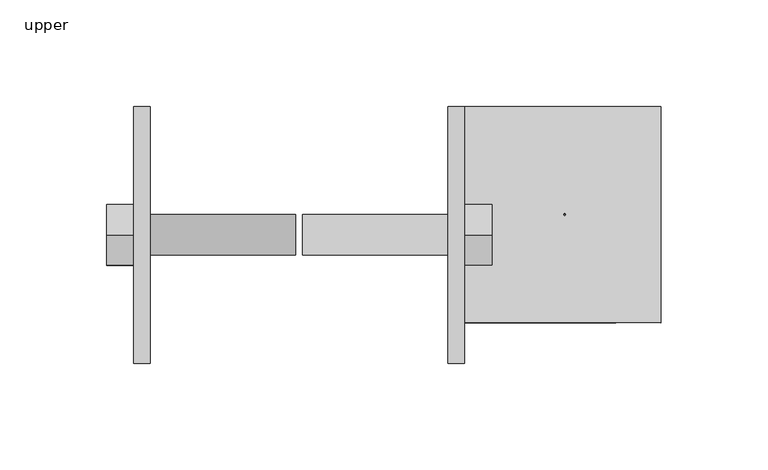
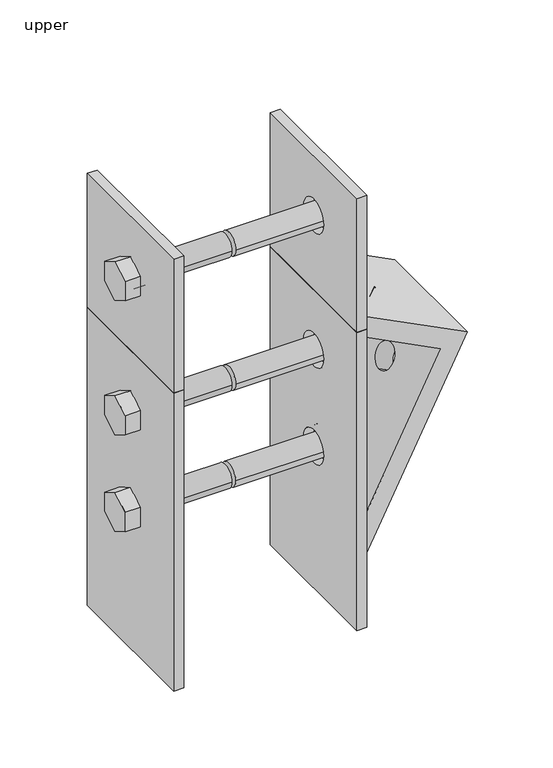
"""IFC4 building model written with IfcOpenShell, lengths in millimetres: fastener geometry, 060523 - W_P_C - Fastenings - Column Base & Top with X Bracing - Custom : upper."""

from ifc_helpers import new_model, si_unit, point, frame, frame_2d, origin, place, context, project, spatial, polyline, circle_curve, trimmed, segment, composite_curve, outline, extrude, source, transform, mapped, element, save
from ifc_brep_helpers import plane_surface, revolved_surface, advanced_brep


def upper_4b50c771(model_context):
    return source(origin(), model_context, "Body", "SolidModel", [
        advanced_brep(
        [(-77.7875, -60.325, 261.9375), (-69.85, -60.325, 261.9375), (-69.85, 60.325, 261.9375), (-77.7875, 60.325, 261.9375), (-77.7875, 52.3875, 261.9375), (-77.7875, 60.325, 7.9375), (-77.7875, 52.3875, 7.9375), (-77.7875, -60.325, 7.9375), (-77.7875, 13.890625, 211.1375), (-77.7875, -13.890625, 211.1375), (-77.7875, 13.890625, 128.5875), (-77.7875, -13.890625, 128.5875), (-69.85, -60.325, 7.9375), (-69.85, 60.325, 7.9375), (-69.85, -13.890625, 211.1375), (-69.85, 13.890625, 211.1375), (-69.85, -13.890625, 128.5875), (-69.85, 13.890625, 128.5875)],
        [
            (0, 1),
            (1, 2),
            (2, 3),
            (3, 4),
            (4, 0),
            (3, 5),
            (5, 6),
            (6, 7),
            (7, 0),
            (8, 9, circle_curve(frame((-77.7875, 0.0, 211.1375), z_axis=(1.0, 0.0, 0.0), x_axis=(0.0, 1.0, 0.0)), 13.890625)),
            (9, 8, circle_curve(frame((-77.7875, 0.0, 211.1375), z_axis=(1.0, 0.0, 0.0), x_axis=(0.0, 1.0, 0.0)), 13.890625)),
            (10, 11, circle_curve(frame((-77.7875, 0.0, 128.5875), z_axis=(1.0, 0.0, 0.0), x_axis=(0.0, 1.0, 0.0)), 13.890625)),
            (11, 10, circle_curve(frame((-77.7875, 0.0, 128.5875), z_axis=(1.0, 0.0, 0.0), x_axis=(0.0, 1.0, 0.0)), 13.890625)),
            (7, 12),
            (12, 1),
            (2, 13),
            (13, 5),
            (14, 15, circle_curve(frame((-69.85, 0.0, 211.1375), z_axis=(1.0, 0.0, 0.0), x_axis=(0.0, 1.0, 0.0)), 13.890625)),
            (15, 8),
            (9, 14),
            (15, 14, circle_curve(frame((-69.85, 0.0, 211.1375), z_axis=(1.0, 0.0, 0.0), x_axis=(0.0, 1.0, 0.0)), 13.890625)),
            (16, 17, circle_curve(frame((-69.85, 0.0, 128.5875), z_axis=(1.0, 0.0, 0.0), x_axis=(0.0, 1.0, 0.0)), 13.890625)),
            (17, 10),
            (11, 16),
            (17, 16, circle_curve(frame((-69.85, 0.0, 128.5875), z_axis=(1.0, 0.0, 0.0), x_axis=(0.0, 1.0, 0.0)), 13.890625)),
            (12, 13),
        ],
        [
            plane_surface(frame((-77.7875, 60.325, 261.9375), z_axis=(0.0, 0.0, 1.0), x_axis=(1.0, 0.0, 0.0))),
            plane_surface(frame((-77.7875, -60.325, 261.9375), z_axis=(-1.0, 0.0, 0.0), x_axis=(0.0, -1.0, 0.0))),
            plane_surface(frame((-77.7875, -60.325, 261.9375), z_axis=(0.0, -1.0, 0.0), x_axis=(1.0, 0.0, 0.0))),
            plane_surface(frame((-77.7875, 60.325, 7.9375), z_axis=(0.0, 1.0, 0.0), x_axis=(1.0, 0.0, 0.0))),
            revolved_surface(polyline([(-77.7875, 13.890625, 211.1375), (-69.85, 13.890625, 211.1375)]), (-69.85, 0.0, 211.1375), (-1.0, 0.0, 0.0)),
            revolved_surface(polyline([(-77.7875, 13.890625, 128.5875), (-69.85, 13.890625, 128.5875)]), (-69.85, 0.0, 128.5875), (-1.0, 0.0, 0.0)),
            plane_surface(frame((-69.85, -60.325, 261.9375), z_axis=(1.0, 0.0, 0.0), x_axis=(0.0, 1.0, 0.0))),
            plane_surface(frame((-77.7875, -60.325, 7.9375), z_axis=(0.0, 0.0, -1.0), x_axis=(1.0, 0.0, 0.0))),
        ],
        [
            (0, [[1, 2, 3, 4, 5]]),
            (1, [[6, 7, 8, 9, -5, -4], [10, 11], [12, 13]]),
            (2, [[14, 15, -1, -9]]),
            (3, [[-3, 16, 17, -6]]),
            (4, [[18, 19, -11, 20]]),
            (4, [[-10, -19, 21, -20]]),
            (5, [[22, 23, -13, 24]]),
            (5, [[-12, -23, 25, -24]]),
            (6, [[-2, -15, 26, -16], [-21, -18], [-25, -22]]),
            (7, [[-17, -26, -14, -8, -7]]),
        ],
    ),
        extrude(outline(polyline([(-14.2875, 219.386392), (0.0, 227.6352839), (14.2875, 219.386392), (14.2875, 202.888608), (0.0, 194.6397161), (-14.2875, 202.888608), (-14.2875, 219.386392)])), frame((-90.4875, 0.0, 0.0), z_axis=(1.0, 0.0, 0.0), x_axis=(0.0, 1.0, 0.0)), (0.0, 0.0, 1.0), 12.7),
        extrude(outline(composite_curve([segment(trimmed(circle_curve(frame_2d((0.0, 211.1375)), 9.525), [point((-9.525, 211.1375))], [point((9.525, 211.1375))], False, "CARTESIAN"), True, "CONTINUOUS"), segment(trimmed(circle_curve(frame_2d((0.0, 211.1375)), 9.525), [point((9.525, 211.1375))], [point((-9.525, 211.1375))], False, "CARTESIAN"), True, "CONTINUOUS")], self_intersect=False)), frame((-77.7875, 0.0, 0.0), z_axis=(1.0, 0.0, 0.0), x_axis=(0.0, 1.0, 0.0)), (0.0, 0.0, 1.0), 76.2),
        extrude(outline(polyline([(-14.2875, 136.836392), (0.0, 145.0852839), (14.2875, 136.836392), (14.2875, 120.338608), (0.0, 112.0897161), (-14.2875, 120.338608), (-14.2875, 136.836392)])), frame((-90.4875, 0.0, 0.0), z_axis=(1.0, 0.0, 0.0), x_axis=(0.0, 1.0, 0.0)), (0.0, 0.0, 1.0), 12.7),
        extrude(outline(composite_curve([segment(trimmed(circle_curve(frame_2d((0.0, 128.5875)), 9.525), [point((-9.525, 128.5875))], [point((9.525, 128.5875))], False, "CARTESIAN"), True, "CONTINUOUS"), segment(trimmed(circle_curve(frame_2d((0.0, 128.5875)), 9.525), [point((9.525, 128.5875))], [point((-9.525, 128.5875))], False, "CARTESIAN"), True, "CONTINUOUS")], self_intersect=False)), frame((-77.7875, 0.0, 0.0), z_axis=(1.0, 0.0, 0.0), x_axis=(0.0, 1.0, 0.0)), (0.0, 0.0, 1.0), 76.2),
        extrude(outline(polyline([(-14.2875, 219.386392), (0.0, 227.6352839), (14.2875, 219.386392), (14.2875, 202.888608), (0.0, 194.6397161), (-14.2875, 202.888608), (-14.2875, 219.386392)])), frame((-90.4875, 0.0, 0.0), z_axis=(1.0, 0.0, 0.0), x_axis=(0.0, 1.0, 0.0)), (0.0, 0.0, 1.0), 12.7),
        extrude(outline(composite_curve([segment(trimmed(circle_curve(frame_2d((0.0, 211.1375)), 9.525), [point((-9.525, 211.1375))], [point((9.525, 211.1375))], False, "CARTESIAN"), True, "CONTINUOUS"), segment(trimmed(circle_curve(frame_2d((0.0, 211.1375)), 9.525), [point((9.525, 211.1375))], [point((-9.525, 211.1375))], False, "CARTESIAN"), True, "CONTINUOUS")], self_intersect=False)), frame((-77.7875, 0.0, 0.0), z_axis=(1.0, 0.0, 0.0), x_axis=(0.0, 1.0, 0.0)), (0.0, 0.0, 1.0), 76.2),
        advanced_brep(
        [(77.7875, -60.325, 261.9375), (77.7875, 52.3875, 261.9375), (77.7875, 60.325, 261.9375), (69.85, 60.325, 261.9375), (69.85, -60.325, 261.9375), (77.7875, -60.325, 7.9375), (77.7875, 52.3875, 7.9375), (77.7875, 60.325, 7.9375), (77.7875, 13.890625, 211.1375), (77.7875, -13.890625, 211.1375), (77.7875, 13.890625, 128.5875), (77.7875, -13.890625, 128.5875), (69.85, -60.325, 7.9375), (69.85, 60.325, 7.9375), (69.85, -13.890625, 211.1375), (69.85, 13.890625, 211.1375), (69.85, -13.890625, 128.5875), (69.85, 13.890625, 128.5875)],
        [
            (0, 1),
            (1, 2),
            (2, 3),
            (3, 4),
            (4, 0),
            (0, 5),
            (5, 6),
            (6, 7),
            (7, 2),
            (8, 9, circle_curve(frame((77.7875, 0.0, 211.1375), z_axis=(-1.0, 0.0, 0.0), x_axis=(0.0, 1.0, 0.0)), 13.890625)),
            (9, 8, circle_curve(frame((77.7875, 0.0, 211.1375), z_axis=(-1.0, 0.0, 0.0), x_axis=(0.0, 1.0, 0.0)), 13.890625)),
            (10, 11, circle_curve(frame((77.7875, 0.0, 128.5875), z_axis=(-1.0, 0.0, 0.0), x_axis=(0.0, 1.0, 0.0)), 13.890625)),
            (11, 10, circle_curve(frame((77.7875, 0.0, 128.5875), z_axis=(-1.0, 0.0, 0.0), x_axis=(0.0, 1.0, 0.0)), 13.890625)),
            (4, 12),
            (12, 5),
            (7, 13),
            (13, 3),
            (14, 9),
            (8, 15),
            (15, 14, circle_curve(frame((69.85, 0.0, 211.1375), z_axis=(-1.0, 0.0, 0.0), x_axis=(0.0, 1.0, 0.0)), 13.890625)),
            (14, 15, circle_curve(frame((69.85, 0.0, 211.1375), z_axis=(-1.0, 0.0, 0.0), x_axis=(0.0, 1.0, 0.0)), 13.890625)),
            (16, 11),
            (10, 17),
            (17, 16, circle_curve(frame((69.85, 0.0, 128.5875), z_axis=(-1.0, 0.0, 0.0), x_axis=(0.0, 1.0, 0.0)), 13.890625)),
            (16, 17, circle_curve(frame((69.85, 0.0, 128.5875), z_axis=(-1.0, 0.0, 0.0), x_axis=(0.0, 1.0, 0.0)), 13.890625)),
            (13, 12),
        ],
        [
            plane_surface(frame((77.7875, 60.325, 261.9375), z_axis=(0.0, 0.0, 1.0), x_axis=(-1.0, 0.0, 0.0))),
            plane_surface(frame((77.7875, -60.325, 261.9375), z_axis=(1.0, 0.0, 0.0), x_axis=(0.0, -1.0, 0.0))),
            plane_surface(frame((77.7875, -60.325, 261.9375), z_axis=(0.0, -1.0, 0.0), x_axis=(-1.0, 0.0, 0.0))),
            plane_surface(frame((77.7875, 60.325, 7.9375), z_axis=(0.0, 1.0, 0.0), x_axis=(-1.0, 0.0, 0.0))),
            revolved_surface(polyline([(77.7875, 13.890625, 211.1375), (69.85, 13.890625, 211.1375)]), (69.85, 0.0, 211.1375), (1.0, 0.0, 0.0)),
            revolved_surface(polyline([(77.7875, 13.890625, 128.5875), (69.85, 13.890625, 128.5875)]), (69.85, 0.0, 128.5875), (1.0, 0.0, 0.0)),
            plane_surface(frame((69.85, -60.325, 261.9375), z_axis=(-1.0, 0.0, 0.0), x_axis=(0.0, 1.0, 0.0))),
            plane_surface(frame((77.7875, -60.325, 7.9375), z_axis=(0.0, 0.0, -1.0), x_axis=(-1.0, 0.0, 0.0))),
        ],
        [
            (0, [[1, 2, 3, 4, 5]]),
            (1, [[-2, -1, 6, 7, 8, 9], [10, 11], [12, 13]]),
            (2, [[-6, -5, 14, 15]]),
            (3, [[-9, 16, 17, -3]]),
            (4, [[18, -10, 19, 20]]),
            (4, [[-18, 21, -19, -11]]),
            (5, [[22, -12, 23, 24]]),
            (5, [[-22, 25, -23, -13]]),
            (6, [[-17, 26, -14, -4], [-20, -21], [-24, -25]]),
            (7, [[-8, -7, -15, -26, -16]]),
        ],
    ),
        extrude(outline(polyline([(-14.2875, 219.386392), (0.0, 227.6352839), (14.2875, 219.386392), (14.2875, 202.888608), (0.0, 194.6397161), (-14.2875, 202.888608), (-14.2875, 219.386392)])), frame((77.7875, 0.0, 0.0), z_axis=(1.0, 0.0, 0.0), x_axis=(0.0, 1.0, 0.0)), (0.0, 0.0, 1.0), 12.7),
        extrude(outline(composite_curve([segment(trimmed(circle_curve(frame_2d((0.0, 211.1375)), 9.525), [point((-9.525, 211.1375))], [point((9.525, 211.1375))], False, "CARTESIAN"), True, "CONTINUOUS"), segment(trimmed(circle_curve(frame_2d((0.0, 211.1375)), 9.525), [point((9.525, 211.1375))], [point((-9.525, 211.1375))], False, "CARTESIAN"), True, "CONTINUOUS")], self_intersect=False)), frame((1.5875, 0.0, 0.0), z_axis=(1.0, 0.0, 0.0), x_axis=(0.0, 1.0, 0.0)), (0.0, 0.0, 1.0), 76.2),
        extrude(outline(polyline([(-14.2875, 136.836392), (0.0, 145.0852839), (14.2875, 136.836392), (14.2875, 120.338608), (0.0, 112.0897161), (-14.2875, 120.338608), (-14.2875, 136.836392)])), frame((77.7875, 0.0, 0.0), z_axis=(1.0, 0.0, 0.0), x_axis=(0.0, 1.0, 0.0)), (0.0, 0.0, 1.0), 12.7),
        extrude(outline(composite_curve([segment(trimmed(circle_curve(frame_2d((0.0, 128.5875)), 9.525), [point((-9.525, 128.5875))], [point((9.525, 128.5875))], False, "CARTESIAN"), True, "CONTINUOUS"), segment(trimmed(circle_curve(frame_2d((0.0, 128.5875)), 9.525), [point((9.525, 128.5875))], [point((-9.525, 128.5875))], False, "CARTESIAN"), True, "CONTINUOUS")], self_intersect=False)), frame((1.5875, 0.0, 0.0), z_axis=(1.0, 0.0, 0.0), x_axis=(0.0, 1.0, 0.0)), (0.0, 0.0, 1.0), 76.2),
        extrude(outline(polyline([(-14.2875, 219.386392), (0.0, 227.6352839), (14.2875, 219.386392), (14.2875, 202.888608), (0.0, 194.6397161), (-14.2875, 202.888608), (-14.2875, 219.386392)])), frame((77.7875, 0.0, 0.0), z_axis=(1.0, 0.0, 0.0), x_axis=(0.0, 1.0, 0.0)), (0.0, 0.0, 1.0), 12.7),
        extrude(outline(composite_curve([segment(trimmed(circle_curve(frame_2d((0.0, 211.1375)), 9.525), [point((-9.525, 211.1375))], [point((9.525, 211.1375))], False, "CARTESIAN"), True, "CONTINUOUS"), segment(trimmed(circle_curve(frame_2d((0.0, 211.1375)), 9.525), [point((9.525, 211.1375))], [point((-9.525, 211.1375))], False, "CARTESIAN"), True, "CONTINUOUS")], self_intersect=False)), frame((1.5875, 0.0, 0.0), z_axis=(1.0, 0.0, 0.0), x_axis=(0.0, 1.0, 0.0)), (0.0, 0.0, 1.0), 76.2),
        advanced_brep(
        [(-77.7875, 60.325, 376.2375), (-77.7875, 60.325, 261.9375), (-77.7875, -52.3875, 261.9375), (-77.7875, -60.325, 261.9375), (-77.7875, -60.325, 376.2375), (-77.7875, 13.890625, 325.4375), (-77.7875, -13.890625, 325.4375), (-69.85, -60.325, 376.2375), (-69.85, 60.325, 376.2375), (-69.85, -60.325, 261.9375), (-69.85, 60.325, 261.9375), (-69.85, -13.890625, 325.4375), (-69.85, 13.890625, 325.4375)],
        [
            (0, 1),
            (1, 2),
            (2, 3),
            (3, 4),
            (4, 0),
            (5, 6, circle_curve(frame((-77.7875, 0.0, 325.4375), z_axis=(1.0, 0.0, 0.0), x_axis=(0.0, 1.0, 0.0)), 13.890625)),
            (6, 5, circle_curve(frame((-77.7875, 0.0, 325.4375), z_axis=(1.0, 0.0, 0.0), x_axis=(0.0, 1.0, 0.0)), 13.890625)),
            (4, 7),
            (7, 8),
            (8, 0),
            (3, 9),
            (9, 7),
            (8, 10),
            (10, 1),
            (11, 12, circle_curve(frame((-69.85, 0.0, 325.4375), z_axis=(1.0, 0.0, 0.0), x_axis=(0.0, 1.0, 0.0)), 13.890625)),
            (12, 5),
            (6, 11),
            (12, 11, circle_curve(frame((-69.85, 0.0, 325.4375), z_axis=(1.0, 0.0, 0.0), x_axis=(0.0, 1.0, 0.0)), 13.890625)),
            (9, 10),
        ],
        [
            plane_surface(frame((-77.7875, -60.325, 376.2375), z_axis=(-1.0, 0.0, 0.0), x_axis=(0.0, -1.0, 0.0))),
            plane_surface(frame((-77.7875, 60.325, 376.2375), z_axis=(0.0, 0.0, 1.0), x_axis=(1.0, 0.0, 0.0))),
            plane_surface(frame((-77.7875, -60.325, 376.2375), z_axis=(0.0, -1.0, 0.0), x_axis=(1.0, 0.0, 0.0))),
            plane_surface(frame((-77.7875, 60.325, 261.9375), z_axis=(0.0, 1.0, 0.0), x_axis=(1.0, 0.0, 0.0))),
            revolved_surface(polyline([(-77.7875, 13.890625, 325.4375), (-69.85, 13.890625, 325.4375)]), (-69.85, 0.0, 325.4375), (-1.0, 0.0, 0.0)),
            plane_surface(frame((-69.85, -60.325, 376.2375), z_axis=(1.0, 0.0, 0.0), x_axis=(0.0, 1.0, 0.0))),
            plane_surface(frame((-77.7875, -60.325, 261.9375), z_axis=(0.0, 0.0, -1.0), x_axis=(1.0, 0.0, 0.0))),
        ],
        [
            (0, [[1, 2, 3, 4, 5], [6, 7]]),
            (1, [[8, 9, 10, -5]]),
            (2, [[11, 12, -8, -4]]),
            (3, [[-10, 13, 14, -1]]),
            (4, [[15, 16, -7, 17]]),
            (4, [[-6, -16, 18, -17]]),
            (5, [[-9, -12, 19, -13], [-18, -15]]),
            (6, [[-14, -19, -11, -3, -2]]),
        ],
    ),
        extrude(outline(polyline([(-14.2875, 333.686392), (0.0, 341.9352839), (14.2875, 333.686392), (14.2875, 317.188608), (0.0, 308.9397161), (-14.2875, 317.188608), (-14.2875, 333.686392)])), frame((-90.4875, 0.0, 0.0), z_axis=(1.0, 0.0, 0.0), x_axis=(0.0, 1.0, 0.0)), (0.0, 0.0, 1.0), 12.7),
        extrude(outline(composite_curve([segment(trimmed(circle_curve(frame_2d((0.0, 325.4375)), 9.525), [point((-9.525, 325.4375))], [point((9.525, 325.4375))], False, "CARTESIAN"), True, "CONTINUOUS"), segment(trimmed(circle_curve(frame_2d((0.0, 325.4375)), 9.525), [point((9.525, 325.4375))], [point((-9.525, 325.4375))], False, "CARTESIAN"), True, "CONTINUOUS")], self_intersect=False)), frame((-77.7875, 0.0, 0.0), z_axis=(1.0, 0.0, 0.0), x_axis=(0.0, 1.0, 0.0)), (0.0, 0.0, 1.0), 76.2),
        advanced_brep(
        [(77.7875, 60.325, 376.2375), (77.7875, -60.325, 376.2375), (77.7875, -60.325, 261.9375), (77.7875, -52.3875, 261.9375), (77.7875, 60.325, 261.9375), (77.7875, 13.890625, 325.4375), (77.7875, -13.890625, 325.4375), (69.85, 60.325, 376.2375), (69.85, -60.325, 376.2375), (69.85, -60.325, 261.9375), (69.85, 60.325, 261.9375), (69.85, -13.890625, 325.4375), (69.85, 13.890625, 325.4375)],
        [
            (0, 1),
            (1, 2),
            (2, 3),
            (3, 4),
            (4, 0),
            (5, 6, circle_curve(frame((77.7875, 0.0, 325.4375), z_axis=(-1.0, 0.0, 0.0), x_axis=(0.0, 1.0, 0.0)), 13.890625)),
            (6, 5, circle_curve(frame((77.7875, 0.0, 325.4375), z_axis=(-1.0, 0.0, 0.0), x_axis=(0.0, 1.0, 0.0)), 13.890625)),
            (0, 7),
            (7, 8),
            (8, 1),
            (8, 9),
            (9, 2),
            (4, 10),
            (10, 7),
            (11, 6),
            (5, 12),
            (12, 11, circle_curve(frame((69.85, 0.0, 325.4375), z_axis=(-1.0, 0.0, 0.0), x_axis=(0.0, 1.0, 0.0)), 13.890625)),
            (11, 12, circle_curve(frame((69.85, 0.0, 325.4375), z_axis=(-1.0, 0.0, 0.0), x_axis=(0.0, 1.0, 0.0)), 13.890625)),
            (10, 9),
        ],
        [
            plane_surface(frame((77.7875, -60.325, 376.2375), z_axis=(1.0, 0.0, 0.0), x_axis=(0.0, -1.0, 0.0))),
            plane_surface(frame((77.7875, 60.325, 376.2375), z_axis=(0.0, 0.0, 1.0), x_axis=(-1.0, 0.0, 0.0))),
            plane_surface(frame((77.7875, -60.325, 376.2375), z_axis=(0.0, -1.0, 0.0), x_axis=(-1.0, 0.0, 0.0))),
            plane_surface(frame((77.7875, 60.325, 261.9375), z_axis=(0.0, 1.0, 0.0), x_axis=(-1.0, 0.0, 0.0))),
            revolved_surface(polyline([(77.7875, 13.890625, 325.4375), (69.85, 13.890625, 325.4375)]), (69.85, 0.0, 325.4375), (1.0, 0.0, 0.0)),
            plane_surface(frame((69.85, -60.325, 376.2375), z_axis=(-1.0, 0.0, 0.0), x_axis=(0.0, 1.0, 0.0))),
            plane_surface(frame((77.7875, -60.325, 261.9375), z_axis=(0.0, 0.0, -1.0), x_axis=(-1.0, 0.0, 0.0))),
        ],
        [
            (0, [[1, 2, 3, 4, 5], [6, 7]]),
            (1, [[-1, 8, 9, 10]]),
            (2, [[-2, -10, 11, 12]]),
            (3, [[-5, 13, 14, -8]]),
            (4, [[15, -6, 16, 17]]),
            (4, [[-15, 18, -16, -7]]),
            (5, [[-14, 19, -11, -9], [-17, -18]]),
            (6, [[-4, -3, -12, -19, -13]]),
        ],
    ),
        extrude(outline(polyline([(-14.2875, 333.686392), (0.0, 341.9352839), (14.2875, 333.686392), (14.2875, 317.188608), (0.0, 308.9397161), (-14.2875, 317.188608), (-14.2875, 333.686392)])), frame((77.7875, 0.0, 0.0), z_axis=(1.0, 0.0, 0.0), x_axis=(0.0, 1.0, 0.0)), (0.0, 0.0, 1.0), 12.7),
        extrude(outline(composite_curve([segment(trimmed(circle_curve(frame_2d((0.0, 325.4375)), 9.525), [point((-9.525, 325.4375))], [point((9.525, 325.4375))], False, "CARTESIAN"), True, "CONTINUOUS"), segment(trimmed(circle_curve(frame_2d((0.0, 325.4375)), 9.525), [point((9.525, 325.4375))], [point((-9.525, 325.4375))], False, "CARTESIAN"), True, "CONTINUOUS")], self_intersect=False)), frame((1.5875, 0.0, 0.0), z_axis=(1.0, 0.0, 0.0), x_axis=(0.0, 1.0, 0.0)), (0.0, 0.0, 1.0), 76.2),
        advanced_brep(
        [(170.0383695, -41.275, 215.9775257), (77.7875, -41.275, 262.9816915), (77.7875, -41.275, 245.1647625), (148.6865418, -41.275, 209.0398963), (77.7875, -41.275, 69.8926921), (77.7875, -41.275, 34.925), (170.0383695, 60.325, 215.9775257), (77.7875, 60.325, 34.925), (77.7875, 60.325, 69.8926921), (148.6865418, 60.325, 209.0398963), (77.7875, 60.325, 245.1647625), (77.7875, 60.325, 262.9816915), (125.1288563, 9.525, 238.8600656), (124.4216199, 9.525, 239.2204206), (117.2145207, 9.525, 225.075692), (117.9217571, 9.525, 224.7153371), (137.6957155, 9.525, 187.4691853), (127.9661316, 9.525, 168.3738017), (142.1108602, 9.525, 161.1667025), (151.8404441, 9.525, 180.2620861)],
        [
            (0, 1),
            (1, 2),
            (2, 3),
            (3, 4),
            (4, 5),
            (5, 0),
            (6, 7),
            (7, 8),
            (8, 9),
            (9, 10),
            (10, 11),
            (11, 6),
            (0, 6),
            (11, 1),
            (12, 13, circle_curve(frame((124.7752381, 9.525, 239.0402431), z_axis=(-0.45399049973954897, 0.0, -0.8910065241883668), x_axis=(-0.8910065241883668, 0.0, 0.45399049973954897)), 0.396875)),
            (13, 12, circle_curve(frame((124.7752381, 9.525, 239.0402431), z_axis=(-0.45399049973954897, 0.0, -0.8910065241883668), x_axis=(-0.8910065241883668, 0.0, 0.45399049973954897)), 0.396875)),
            (10, 2),
            (9, 3),
            (14, 15, circle_curve(frame((117.5681389, 9.525, 224.8955145), z_axis=(0.45399049973954897, 0.0, 0.8910065241883668), x_axis=(-0.8910065241883668, 0.0, 0.45399049973954897)), 0.396875)),
            (15, 14, circle_curve(frame((117.5681389, 9.525, 224.8955145), z_axis=(0.45399049973954897, 0.0, 0.8910065241883668), x_axis=(-0.8910065241883668, 0.0, 0.45399049973954897)), 0.396875)),
            (8, 4),
            (16, 17, circle_curve(frame((132.8309236, 9.525, 177.9214935), z_axis=(0.8910065241883661, 0.0, -0.4539904997395502), x_axis=(0.4539904997395502, 0.0, 0.8910065241883661)), 10.715625)),
            (17, 16, circle_curve(frame((132.8309236, 9.525, 177.9214935), z_axis=(0.8910065241883661, 0.0, -0.4539904997395502), x_axis=(0.4539904997395502, 0.0, 0.8910065241883661)), 10.715625)),
            (7, 5),
            (18, 19, circle_curve(frame((146.9756522, 9.525, 170.7143943), z_axis=(-0.8910065241883661, 0.0, 0.4539904997395502), x_axis=(0.4539904997395502, 0.0, 0.8910065241883661)), 10.715625)),
            (19, 18, circle_curve(frame((146.9756522, 9.525, 170.7143943), z_axis=(-0.8910065241883661, 0.0, 0.4539904997395502), x_axis=(0.4539904997395502, 0.0, 0.8910065241883661)), 10.715625)),
            (12, 15),
            (14, 13),
            (18, 17),
            (16, 19),
        ],
        [
            plane_surface(frame((77.7875, -41.275, 262.9816915), z_axis=(0.0, -1.0, 0.0), x_axis=(-0.8910065241883668, 0.0, 0.45399049973954897))),
            plane_surface(frame((77.7875, 60.325, 262.9816915), z_axis=(0.0, 1.0, 0.0), x_axis=(0.8910065241883668, 0.0, -0.45399049973954897))),
            plane_surface(frame((170.0383695, -41.275, 215.9775257), z_axis=(0.45399049973954897, 0.0, 0.8910065241883668), x_axis=(0.0, 1.0, 0.0))),
            plane_surface(frame((77.7875, -41.275, 262.9816915), z_axis=(-1.0, 0.0, 0.0), x_axis=(0.0, 1.0, 0.0))),
            plane_surface(frame((77.7875, -41.275, 245.1647625), z_axis=(-0.4539904997395488, 0.0, -0.8910065241883668), x_axis=(0.0, 1.0, 0.0))),
            plane_surface(frame((148.6865418, -41.275, 209.0398963), z_axis=(-0.8910065241883659, 0.0, 0.45399049973955063), x_axis=(0.0, 1.0, 0.0))),
            plane_surface(frame((77.7875, -41.275, 69.8926921), z_axis=(-1.0, 0.0, 0.0), x_axis=(0.0, 1.0, 0.0))),
            plane_surface(frame((77.7875, -41.275, 34.925), z_axis=(0.8910065241883661, 0.0, -0.4539904997395502), x_axis=(0.0, 1.0, 0.0))),
            revolved_surface(polyline([(117.21452068738647, 9.525, 225.0756919787313), (124.42161989691586, 9.525, 239.22042060157148)]), (124.7752381, 9.525, 239.0402431), (-0.45399049973954897, 0.0, -0.8910065241883668)),
            revolved_surface(polyline([(137.69571550343758, 9.525, 187.4691853067466), (151.84044414877164, 9.525, 180.26208608575598)]), (146.9756522, 9.525, 170.7143943), (-0.8910065241883661, 0.0, 0.4539904997395502)),
        ],
        [
            (0, [[1, 2, 3, 4, 5, 6]]),
            (1, [[7, 8, 9, 10, 11, 12]]),
            (2, [[-1, 13, -12, 14], [15, 16]]),
            (3, [[-2, -14, -11, 17]]),
            (4, [[-3, -17, -10, 18], [19, 20]]),
            (5, [[-4, -18, -9, 21], [22, 23]]),
            (6, [[-5, -21, -8, 24]]),
            (7, [[-6, -24, -7, -13], [25, 26]]),
            (8, [[27, -19, 28, -15]]),
            (8, [[-27, -16, -28, -20]]),
            (9, [[29, -22, 30, -25]]),
            (9, [[-29, -26, -30, -23]]),
        ],
    ),
    ])


if __name__ == "__main__":
    model = new_model("IFC4")
    model_context = context("Model", 3, world=origin())
    ifc_project = project(units=[si_unit("LENGTHUNIT", "METRE", prefix="MILLI")], contexts=[model_context])
    site = spatial("IfcSite", under=ifc_project)
    building = spatial("IfcBuilding", under=site)
    placement = place(None, origin())
    upper_shape = upper_4b50c771(model_context)
    element("IfcFastener", 1, ObjectType="060523 - W_P_C - Fastenings - Column Base & Top with X Bracing - Custom : upper", at=placement, inside=building, context=model_context, shape_type="MappedRepresentation", body=[
        mapped(upper_shape, transform((0.0, 0.0, 0.0), x_axis=(1.0, 0.0, 0.0), y_axis=(0.0, 1.0, 0.0), z_axis=(0.0, 0.0, 1.0))),
    ])
    save(model, "model.ifc")

# Revit data of these elements
# Type "060523 - W_P_C - Fastenings - Column Base & Top with X Bracing - Custom : upper"
#   Width - Top = 0' - 5 1/2"
#   Top/Bottom Plate Thickness = 0' - 0 5/16"
#   Top/Bottom Plate - Width = 0' - 7 1/2"
#   Rod Radius = 0' - 0 3/8"
#   Rod Length [instance default] = 1' - 0"
#   Plate Thickness = 0' - 0 5/16"
#   Offset - Upper Plate 2 = 0' - 0"
#   Height of Plate = 0' - 10"
#   Width - Bottom = 0' - 5 1/2"
#   Plate Width = 0' - 4 3/4"
#   Bracket Width = 0' - 4"
#   Bracket Thickness = 0' - 0 5/8"
#   Bracket Offset in X = 0' - 3 1/16"
#   Bracket Offset in Y = 0' - 0"
#   Bracket Offset = 0' - 1 3/8"
#   Bracket Leg = 0' - 8"
#   Bracket Hole Radius - Up = 0' - 0 1/64"
#   Bracket Hole Radius - Down = 0' - 0 27/64"
#   Bracket Hole Offset = 0' - 2"
#   Beam Width = 0' - 7 3/8"
#   Angle 2 = 63.00°
#   Angle 1 = 153.00°
#   Top Plate Visible = no
#   Rod Visibility = no
#   Plate Visibility - Upper Right 2 = no
#   Plate Visibility - Upper Right 1 = yes
#   Plate Visibility - Upper Left 2 = no
#   Plate Visibility - Upper Left 1 = yes
#   Plate Visibility - Lower Right 2 = no
#   Plate Visibility - Lower Right 1 = yes
#   Plate Visibility - Lower Left 2 = no
#   Plate Visibility - Lower Left 1 = yes
#   Bracket Visibility = yes
#   Bottom Plate Visible = no
#   Upper Plates - 2 = element 1925096
#   Upper Plates - 1 = element 1925090
#   Rod Material = 3/4" STEEL (RAW) ROD (THREADED AT ENDS) - W/ TURNBUCKLE
#   Lower Plates = element 1925094
#   Bracket Material = 5/8" STEEL ANGLE (RAW STEEL)
#   URL = ""
# Element 1 (IfcFastener, "060523 - W_P_C - Fastenings - Column Base & Top with X Bracing - Custom : upper")
#   Rod Length = 11' - 3"
#   Materials on its faces: "3/4\" LAG BOLT (THRU BOLT IF PLATE ON OPP. SIDE OF STRUCT MEMBER)", "5/16\" STEEL PLATE (RAW STEEL)", "5/8\" STEEL ANGLE (RAW STEEL)"
# Materials
#   "3/4\" STEEL (RAW) ROD (THREADED AT ENDS) - W/ TURNBUCKLE": class "Generic", colour RGB 120 120 120, transparency 0, Cost = 0
#   "5/8\" STEEL ANGLE (RAW STEEL)": class "Generic", colour RGB 195 195 195, transparency 0, Cost = 0
#   "3/4\" LAG BOLT (THRU BOLT IF PLATE ON OPP. SIDE OF STRUCT MEMBER)": class "Generic", colour RGB 120 120 120, transparency 0, Cost = 0
#   "5/16\" STEEL PLATE (RAW STEEL)": class "Generic", colour RGB 232 232 232, transparency 0, Cost = 0
